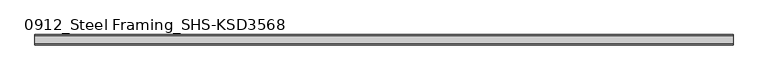
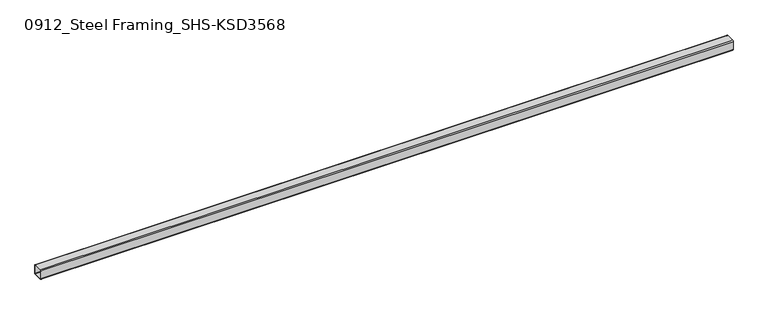
"""IFC4 building model written with IfcOpenShell, lengths in millimetres: beam geometry, 0912_Steel Framing_SHS-KSD3568 : H_SB_ASB_SHS-150x150x6."""

from ifc_helpers import new_model, si_unit, point, frame, frame_2d, origin, place, context, project, spatial, polyline, circle_curve, trimmed, segment, composite_curve, outline, extrude, source, transform, mapped, element, save


def beam_0912_steel_framing_shs_ksd3568_e5cce134(model_context):
    return source(origin(), model_context, "Body", "SweptSolid", [
        extrude(outline(composite_curve([segment(trimmed(circle_curve(frame_2d((-63.0, 63.0)), 12.0), [point((-75.0, 63.0))], [point((-63.0, 75.0))], False, "CARTESIAN"), True, "CONTINUOUS"), segment(polyline([(-63.0, 75.0), (63.0, 75.0)]), True, "CONTINUOUS"), segment(trimmed(circle_curve(frame_2d((63.0, 63.0)), 12.0), [point((63.0, 75.0))], [point((75.0, 63.0))], False, "CARTESIAN"), True, "CONTINUOUS"), segment(polyline([(75.0, 63.0), (75.0, -63.0)]), True, "CONTINUOUS"), segment(trimmed(circle_curve(frame_2d((63.0, -63.0)), 12.0), [point((75.0, -63.0))], [point((63.0, -75.0))], False, "CARTESIAN"), True, "CONTINUOUS"), segment(polyline([(63.0, -75.0), (-63.0, -75.0)]), True, "CONTINUOUS"), segment(trimmed(circle_curve(frame_2d((-63.0, -63.0)), 12.0), [point((-63.0, -75.0))], [point((-75.0, -63.0))], False, "CARTESIAN"), True, "CONTINUOUS"), segment(polyline([(-75.0, -63.0), (-75.0, 63.0)]), True, "CONTINUOUS")], self_intersect=False), holes=[composite_curve([segment(polyline([(63.0, 69.0), (-63.0, 69.0)]), True, "CONTINUOUS"), segment(trimmed(circle_curve(frame_2d((-63.0, 63.0)), 6.0), [point((-63.0, 69.0))], [point((-69.0, 63.0))], True, "CARTESIAN"), True, "CONTINUOUS"), segment(polyline([(-69.0, 63.0), (-69.0, -63.0)]), True, "CONTINUOUS"), segment(trimmed(circle_curve(frame_2d((-63.0, -63.0)), 6.0), [point((-69.0, -63.0))], [point((-63.0, -69.0))], True, "CARTESIAN"), True, "CONTINUOUS"), segment(polyline([(-63.0, -69.0), (63.0, -69.0)]), True, "CONTINUOUS"), segment(trimmed(circle_curve(frame_2d((63.0, -63.0)), 6.0), [point((63.0, -69.0))], [point((69.0, -63.0))], True, "CARTESIAN"), True, "CONTINUOUS"), segment(polyline([(69.0, -63.0), (69.0, 63.0)]), True, "CONTINUOUS"), segment(trimmed(circle_curve(frame_2d((63.0, 63.0)), 6.0), [point((69.0, 63.0))], [point((63.0, 69.0))], True, "CARTESIAN"), True, "CONTINUOUS")], self_intersect=False)]), frame((-5049.8, 0.0, 0.0), z_axis=(1.0, 0.0, 0.0), x_axis=(0.0, 1.0, 0.0)), (0.0, 0.0, 1.0), 10224.6),
    ])


if __name__ == "__main__":
    model = new_model("IFC4")
    model_context = context("Model", 3, world=origin())
    ifc_project = project(units=[si_unit("LENGTHUNIT", "METRE", prefix="MILLI")], contexts=[model_context])
    site = spatial("IfcSite", under=ifc_project)
    building = spatial("IfcBuilding", under=site)
    placement = place(None, origin())
    beam_0912_steel_framing_shs_ksd3568_shape = beam_0912_steel_framing_shs_ksd3568_e5cce134(model_context)
    element("IfcBeam", 1, ObjectType="0912_Steel Framing_SHS-KSD3568 : H_SB_ASB_SHS-150x150x6", at=placement, inside=building, context=model_context, shape_type="MappedRepresentation", body=[
        mapped(beam_0912_steel_framing_shs_ksd3568_shape, transform((0.0, 0.0, 0.0), x_axis=(1.0, 0.0, 0.0), y_axis=(0.0, 1.0, 0.0), z_axis=(0.0, 0.0, 1.0))),
    ])
    save(model, "model.ifc")

# Revit data of these elements
# Type "0912_Steel Framing_SHS-KSD3568 : H_SB_ASB_SHS-150x150x6"
#   H_WM Code_1 = "S01AA002-00001 | Main Steel Structure Fabrication Work | Shelter/Building | Medium Steel - Standard (90KG/M>Weight≥30KG/M) | Material: (   )"
#   H_WM Code_2 = "S03AA028-00001 | Main Steel Structure Erection Work | Shelter/Building | Medium Steel (90KG/M>Weight≥30KG/M) | Material: (   )"
#   H_WM Code_3 = "S01AA010-00001 | Main Steel Structure Fabrication Work | Shelter/Building | Steel Painting/Coating | for Non-Fireproofed Steel Surface, Surface Preparation, Primer, Second & Final Coat | Material: (   )"
#   H_Q'ty Cal Type Tag = "SB-Q2"
#   Perimeter = 0.60 m²/m
#   Nominal Weight = 26.40 kgf/m
#   Length [instance default] = 1.0000 m
#   b = 0.1500 m
#   h = 0.1500 m
#   tr = 0.0120 m
#   t = 0.0060 m
#   A = 28.36 m²
#   Structural Material [instance default] = Steel, 45-345
# Element 1 (IfcBeam, "0912_Steel Framing_SHS-KSD3568 : H_SB_ASB_SHS-150x150x6")
#   Structural Material = none
# Materials
#   "Steel, 45-345": class "Metal", colour RGB 189 187 185, transparency 0, Description = "Steel 345 MPa", Cost = 0
